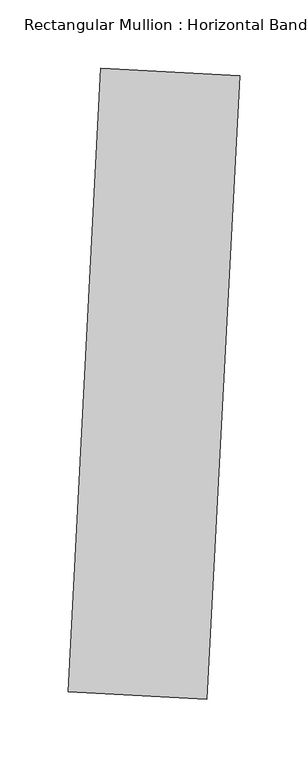
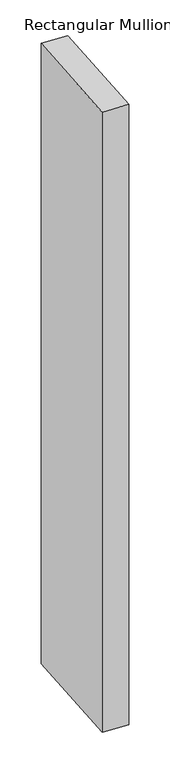
"""IFC4 building model written with IfcOpenShell, lengths in millimetres: member geometry, Rectangular Mullion : Horizontal Band."""

from ifc_helpers import new_model, si_unit, frame, origin, place, context, project, spatial, polyline, outline, extrude, source, transform, mapped, element, save


def rectangular_mullion_horizontal_band_466c517c(model_context):
    return source(origin(), model_context, "Body", "SweptSolid", [
        extrude(outline(polyline([(62.69438, 301.8280451), (38.7663808, -154.7453782), (-62.69438, -149.4280451), (-38.7663808, 307.1453782), (62.69438, 301.8280451)])), frame((0.0, 0.0, -2573.7181637), z_axis=(0.0, 0.0, 1.0), x_axis=(1.0, 0.0, 0.0)), (0.0, 0.0, 1.0), 2573.7181637),
    ])


if __name__ == "__main__":
    model = new_model("IFC4")
    model_context = context("Model", 3, world=origin())
    ifc_project = project(units=[si_unit("LENGTHUNIT", "METRE", prefix="MILLI")], contexts=[model_context])
    site = spatial("IfcSite", under=ifc_project)
    building = spatial("IfcBuilding", under=site)
    placement = place(None, origin())
    rectangular_mullion_horizontal_band_shape = rectangular_mullion_horizontal_band_466c517c(model_context)
    element("IfcMember", 1, ObjectType="Rectangular Mullion : Horizontal Band", at=placement, inside=building, context=model_context, shape_type="MappedRepresentation", body=[
        mapped(rectangular_mullion_horizontal_band_shape, transform((0.0, 0.0, 0.0), x_axis=(1.0, 0.0, 0.0), y_axis=(0.0, 1.0, 0.0), z_axis=(0.0, 0.0, 1.0))),
    ])
    save(model, "model.ifc")

# Revit data of these elements
# Type "Rectangular Mullion : Horizontal Band"
#   built-in parameter 1007351 = 0.25 (stored number, unit not read)
#   built-in parameter 1007304 = 1.5 (stored number, unit not read)
#   built-in parameter 1007301 = 0.166667 (stored number, unit not read)
#   built-in parameter 1007300 = 0.166667 (stored number, unit not read)
# Element 1 (IfcMember, "Rectangular Mullion : Horizontal Band")
#   Materials on its faces: "Aluminum"
# Materials
#   "Aluminum": class "Metal", colour RGB 247 247 247, transparency 0, Description = "Aluminum 6061", Cost = 0
